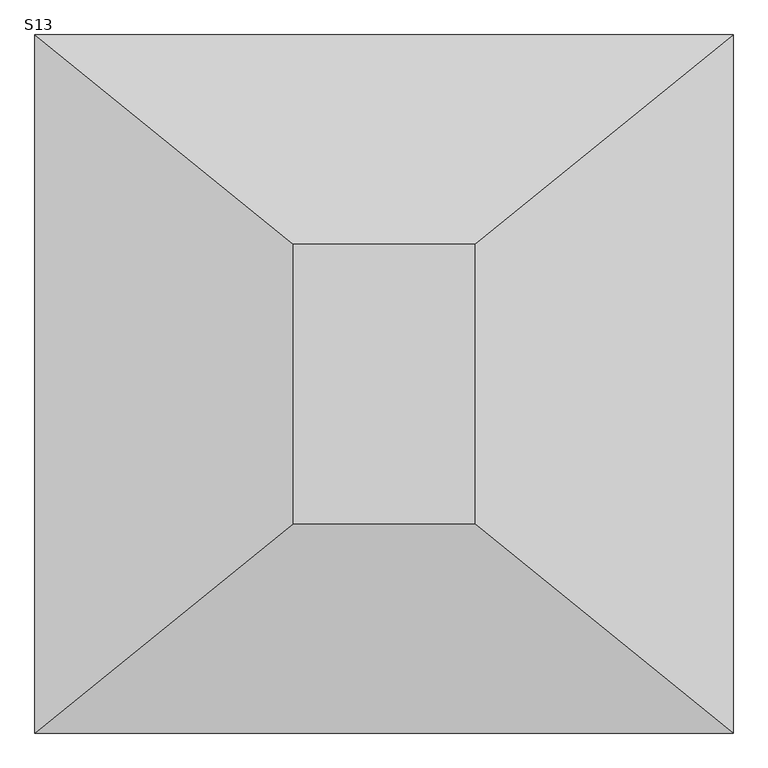
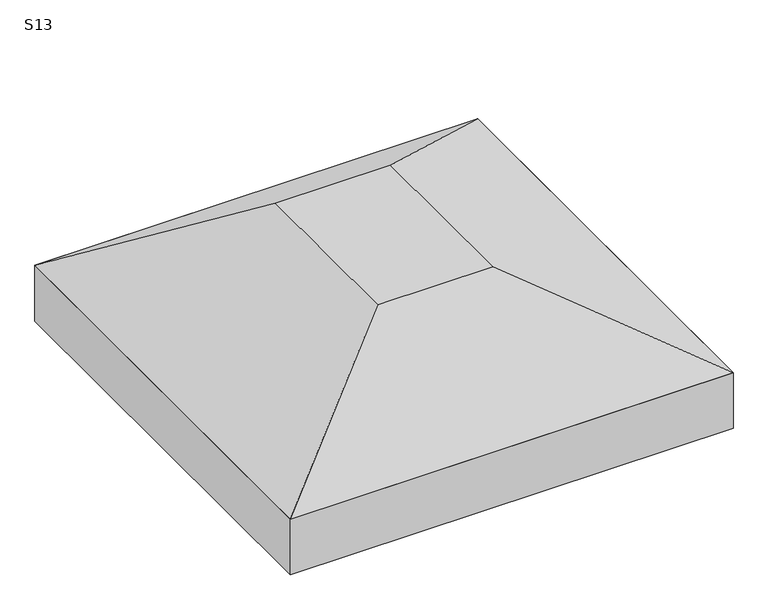
"""IFC4 building model written with IfcOpenShell, lengths in millimetres: fastener geometry, TQS - Sapata : S13."""

from ifc_helpers import new_model, si_unit, frame, origin, place, context, project, spatial, polyline, outline, extrude, faceted_brep, source, transform, mapped, element, save


def s13_7eae1afe(model_context):
    return source(origin(), model_context, "Body", "SolidModel", [
        faceted_brep([(-5.0, 100.0, 0.0), (-395.0, 100.0, 0.0), (-395.0, -500.0, 0.0), (-5.0, -500.0, 0.0), (550.0, 550.0, -300.0), (550.0, -950.0, -300.0), (-950.0, -950.0, -300.0), (-950.0, 550.0, -300.0)], [[[0, 1, 2, 3]], [[4, 5, 6, 7]], [[4, 7, 1, 0]], [[7, 6, 2, 1]], [[6, 5, 3, 2]], [[5, 4, 0, 3]]]),
        extrude(outline(polyline([(550.0, 550.0), (550.0, -950.0), (-950.0, -950.0), (-950.0, 550.0), (550.0, 550.0)])), frame((0.0, 0.0, -500.0), z_axis=(0.0, 0.0, 1.0), x_axis=(1.0, 0.0, 0.0)), (0.0, 0.0, 1.0), 200.0),
    ])


if __name__ == "__main__":
    model = new_model("IFC4")
    model_context = context("Model", 3, world=origin())
    ifc_project = project(units=[si_unit("LENGTHUNIT", "METRE", prefix="MILLI")], contexts=[model_context])
    site = spatial("IfcSite", under=ifc_project)
    building = spatial("IfcBuilding", under=site)
    placement = place(None, origin())
    s13_shape = s13_7eae1afe(model_context)
    element("IfcFastener", 1, ObjectType="TQS - Sapata : S13", at=placement, inside=building, context=model_context, shape_type="MappedRepresentation", body=[
        mapped(s13_shape, transform((0.0, 0.0, 0.0), x_axis=(1.0, 0.0, 0.0), y_axis=(0.0, 1.0, 0.0), z_axis=(0.0, 0.0, 1.0))),
    ])
    save(model, "model.ifc")

# Revit data of these elements
# Type "TQS - Sapata : S13"
#   TY = 0.60 m
#   TX = 0.39 m
#   HS = 0.50 m
#   H0 = 0.20 m
#   EXCYABS = 0.75 m
#   EXCY = 0.00 m
#   EXCXABS = 0.75 m
#   EXCX = 0.00 m
#   DIMY = 1.50 m
#   DIMX = 1.50 m
#   Material estrutural = Concreto - Concreto concretado no local
#   Width = 0
#   Length = 0
# Element 1 (IfcFastener, "TQS - Sapata : S13")
#   Materials on its faces: "Concreto - Concreto concretado no local"
# Materials
#   "Concreto - Concreto concretado no local": class "Concreto", colour RGB 192 192 192, transparency 0
